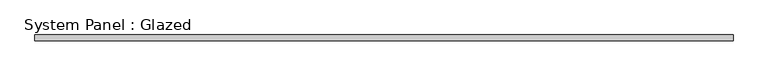
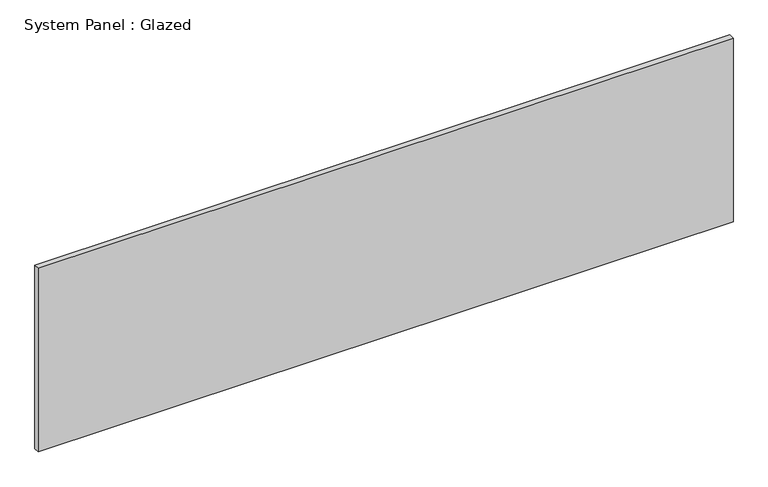
"""IFC4 building model written with IfcOpenShell, lengths in millimetres: plate geometry, System Panel : Glazed."""

import ifcopenshell
import ifcopenshell.guid

model = None  # the IFC model being written
_history = None  # IfcOwnerHistory: only IFC2X3 demands one
_inside = {}  # id of a spatial element -> (the spatial element, [elements in it])
_under = {}  # id of a project, library or spatial element -> (it, [spatial elements below it])
_declared = {}  # id of a project -> (the project, [libraries it declares])
_typed = {}  # id of a type object -> (the type object, [elements of that type])
_made_of = {}  # id of a material, layer set ... -> (it, [elements and type objects made of it])


def new_model(schema):
    """Start an empty IFC model of exactly this schema.

    Asked for "IFC4X3", IfcOpenShell would pick the latest addendum, in which some entities
    have other attributes; the version numbers below select the first issue.
    IFC2X3 requires an IfcOwnerHistory on every rooted entity: one is made here for all.
    """
    global model, _history
    if schema == "IFC4X3":
        model = ifcopenshell.file(schema_version=(4, 3, 0, 0))
    else:
        model = ifcopenshell.file(schema=schema)
    _inside.clear()
    _under.clear()
    _declared.clear()
    _typed.clear()
    _made_of.clear()
    _history = None
    if model.schema == "IFC2X3":
        org = make("IfcOrganization", Name="unknown")
        user = make(
            "IfcPersonAndOrganization",
            ThePerson=make("IfcPerson", FamilyName="unknown"),
            TheOrganization=org,
        )
        app = make(
            "IfcApplication",
            ApplicationDeveloper=org,
            Version="unknown",
            ApplicationFullName="unknown",
            ApplicationIdentifier="unknown",
        )
        _history = make(
            "IfcOwnerHistory",
            OwningUser=user,
            OwningApplication=app,
            ChangeAction="ADDED",
            CreationDate=0,
        )
    return model


def make(cls, **values):
    """One entity of the class cls with the attributes given. An attribute that is None is left unset."""
    return model.create_entity(
        cls, **{name: value for name, value in values.items() if value is not None}
    )


def rooted(cls, **values):
    """An entity with a GlobalId (a new one), such as an element, a storey or a relation."""
    return make(cls, GlobalId=ifcopenshell.guid.new(), OwnerHistory=_history, **values)


def si_unit(unit_type, name, prefix=None):
    """IfcSIUnit, for example si_unit("LENGTHUNIT", "METRE", prefix="MILLI")."""
    return make("IfcSIUnit", UnitType=unit_type, Prefix=prefix, Name=name)


def assignment(units):
    """IfcUnitAssignment: the units of a project."""
    return None if units is None else make("IfcUnitAssignment", Units=units)


def point(xyz):
    """IfcCartesianPoint."""
    return None if xyz is None else make("IfcCartesianPoint", Coordinates=xyz)


def direction(xyz):
    """IfcDirection."""
    return None if xyz is None else make("IfcDirection", DirectionRatios=xyz)


def frame(location, z_axis=None, x_axis=None):
    """IfcAxis2Placement3D, a coordinate frame: its origin and axes. An axis left out is left unset."""
    return make(
        "IfcAxis2Placement3D",
        Location=point(location),
        Axis=direction(z_axis),
        RefDirection=direction(x_axis),
    )


def origin():
    """The frame at (0, 0, 0) with its axes left unset."""
    return frame((0.0, 0.0, 0.0))


def origin_with_axes():
    """The frame at (0, 0, 0) with the z axis (0, 0, 1) and the x axis (1, 0, 0) written out."""
    return frame((0.0, 0.0, 0.0), z_axis=(0.0, 0.0, 1.0), x_axis=(1.0, 0.0, 0.0))


def place(relative_to, where):
    """IfcLocalPlacement: puts the frame where relative to a parent placement (None: the world)."""
    return make(
        "IfcLocalPlacement", PlacementRelTo=relative_to, RelativePlacement=where
    )


def context(
    kind, dimensions, precision=None, world=None, true_north=None, identifier=None
):
    """IfcGeometricRepresentationContext, for example the 3D "Model" context."""
    return make(
        "IfcGeometricRepresentationContext",
        ContextIdentifier=identifier,
        ContextType=kind,
        CoordinateSpaceDimension=dimensions,
        Precision=precision,
        WorldCoordinateSystem=world,
        TrueNorth=true_north,
    )


def project(units=None, contexts=None):
    """IfcProject with its units and contexts."""
    return rooted(
        "IfcProject",
        Name="project",
        RepresentationContexts=contexts,
        UnitsInContext=assignment(units),
    )


def spatial(cls, under=None, at=None, **own):
    """A site, building, storey or space (cls), placed at a placement, below another one or the project."""
    s = rooted(cls, ObjectPlacement=at, **own)
    if under is not None:
        _under.setdefault(under.id(), (under, []))[1].append(s)
    return s


def polyline(points):
    """IfcPolyline through the points."""
    return make("IfcPolyline", Points=[point(p) for p in points])


def outline(outer, holes=None, kind="AREA"):
    """IfcArbitraryClosedProfileDef: a profile drawn as a closed curve; with holes, ...WithVoids."""
    if holes is None:
        return make("IfcArbitraryClosedProfileDef", ProfileType=kind, OuterCurve=outer)
    return make(
        "IfcArbitraryProfileDefWithVoids",
        ProfileType=kind,
        OuterCurve=outer,
        InnerCurves=holes,
    )


def extrude(swept, where, along, depth):
    """IfcExtrudedAreaSolid: the profile swept, set in the frame where, extruded along a direction by depth."""
    return make(
        "IfcExtrudedAreaSolid",
        SweptArea=swept,
        Position=where,
        ExtrudedDirection=direction(along),
        Depth=depth,
    )


def shape(context_of_items, identifier, shape_type, items):
    """IfcShapeRepresentation: the items that make up one representation, for example the "Body"."""
    return make(
        "IfcShapeRepresentation",
        ContextOfItems=context_of_items,
        RepresentationIdentifier=identifier,
        RepresentationType=shape_type,
        Items=items,
    )


def source(mapping_origin, context_of_items, identifier, shape_type, items):
    """IfcRepresentationMap: a shape defined once, which mapped items show again and again."""
    return make(
        "IfcRepresentationMap",
        MappingOrigin=mapping_origin,
        MappedRepresentation=shape(context_of_items, identifier, shape_type, items),
    )


def transform(
    local_origin,
    x_axis=None,
    y_axis=None,
    z_axis=None,
    scale=None,
    scale2=None,
    scale3=None,
    uniform=True,
):
    """IfcCartesianTransformationOperator3D, or its non-uniform kind. x_axis, y_axis, z_axis: its Axis1, 2, 3."""
    if uniform:
        return make(
            "IfcCartesianTransformationOperator3D",
            Axis1=direction(x_axis),
            Axis2=direction(y_axis),
            LocalOrigin=point(local_origin),
            Scale=scale,
            Axis3=direction(z_axis),
        )
    return make(
        "IfcCartesianTransformationOperator3DnonUniform",
        Axis1=direction(x_axis),
        Axis2=direction(y_axis),
        LocalOrigin=point(local_origin),
        Scale=scale,
        Axis3=direction(z_axis),
        Scale2=scale2,
        Scale3=scale3,
    )


def mapped(mapping_source, mapping_target):
    """IfcMappedItem: shows the shape of a source again, moved by a transform."""
    return make(
        "IfcMappedItem", MappingSource=mapping_source, MappingTarget=mapping_target
    )


def made_of(thing, what):
    """Note that an element or type object is made of a material, layer set ...; save() writes the relation."""
    if what is not None:
        _made_of.setdefault(what.id(), (what, []))[1].append(thing)
    return thing


def element(
    cls,
    number,
    at=None,
    inside=None,
    cuts=None,
    type_object=None,
    material=None,
    context=None,
    identifier="Body",
    shape_type=None,
    held_by="IfcProductDefinitionShape",
    body=None,
    shapes=None,
    **own,
):
    """One element of the class cls, such as IfcWall. Its Tag is "e" and its number.

    at: its placement. inside: the storey or other place that contains it. cuts: it is an
    opening in that element (IfcRelVoidsElement). A single representation is given by context,
    identifier, shape_type and body (its items); several are given by shapes. held_by: the class
    of the entity that holds the representations. save() writes the other relations.
    """
    e = rooted(cls, Tag="e%d" % number, ObjectPlacement=at, **own)
    if body is not None:
        shapes = [shape(context, identifier, shape_type, body)]
    if shapes is not None:
        e.Representation = make(held_by, Representations=shapes)
    if inside is not None:
        _inside.setdefault(inside.id(), (inside, []))[1].append(e)
    if cuts is not None:
        rooted(
            "IfcRelVoidsElement", RelatingBuildingElement=cuts, RelatedOpeningElement=e
        )
    if type_object is not None:
        _typed.setdefault(type_object.id(), (type_object, []))[1].append(e)
    return made_of(e, material)


def aggregate(whole, parts):
    """IfcRelAggregates: a whole, such as a stair, and the parts it consists of."""
    return rooted("IfcRelAggregates", RelatingObject=whole, RelatedObjects=parts)


def save(model, path):
    """Write the relations noted so far, then the file.

    IfcRelAggregates (storeys below a building ...), IfcRelContainedInSpatialStructure (elements
    in a storey), IfcRelDefinesByType, IfcRelAssociatesMaterial and IfcRelDeclares: one each for
    every whole, place, type object, material and project.
    """
    for whole, parts in _under.values():
        aggregate(whole, parts)
    for where, things in _inside.values():
        rooted(
            "IfcRelContainedInSpatialStructure",
            RelatedElements=things,
            RelatingStructure=where,
        )
    for kind, things in _typed.values():
        rooted("IfcRelDefinesByType", RelatedObjects=things, RelatingType=kind)
    for what, things in _made_of.values():
        rooted("IfcRelAssociatesMaterial", RelatedObjects=things, RelatingMaterial=what)
    for by, libraries in _declared.values():
        rooted("IfcRelDeclares", RelatingContext=by, RelatedDefinitions=libraries)
    model.write(path)


def system_panel_glazed_495097d9(model_context):
    return source(origin(), model_context, "Body", "SweptSolid", [
        extrude(outline(polyline([(1549.4, -44.45), (-1549.4, -44.45), (-1549.4, -19.05), (1549.4, -19.05), (1549.4, -44.45)])), origin_with_axes(), (0.0, 0.0, 1.0), 866.081558),
    ])


if __name__ == "__main__":
    model = new_model("IFC4")
    model_context = context("Model", 3, world=origin())
    ifc_project = project(units=[si_unit("LENGTHUNIT", "METRE", prefix="MILLI")], contexts=[model_context])
    site = spatial("IfcSite", under=ifc_project)
    building = spatial("IfcBuilding", under=site)
    placement = place(None, origin())
    system_panel_glazed_shape = system_panel_glazed_495097d9(model_context)
    element("IfcPlate", 1, ObjectType="System Panel : Glazed", at=placement, inside=building, context=model_context, shape_type="MappedRepresentation", body=[
        mapped(system_panel_glazed_shape, transform((0.0, 0.0, 0.0), x_axis=(1.0, 0.0, 0.0), y_axis=(0.0, 1.0, 0.0), z_axis=(0.0, 0.0, 1.0))),
    ])
    save(model, "model.ifc")

# Revit data of these elements
# Type "System Panel : Glazed"
#   Construction Type Id = "GSP4R"
#   Analytic Construction = "1/8 in Pilkington single glazing"
#   Visual Light Transmittance = 0.9
#   Solar Heat Gain Coefficient = 0.86
#   Heat Transfer Coefficient (U) = 1.18115 BTU/(h·ft²·°F)
#   Define Thermal Properties by = 1
# Element 1 (IfcPlate, "System Panel : Glazed")
#   Materials on its faces: "Glass"
# Materials
#   "Glass": class "Glass", colour RGB 0 128 192, transparency 0.75, Description = "Soda Lime Glass", Cost = 0
